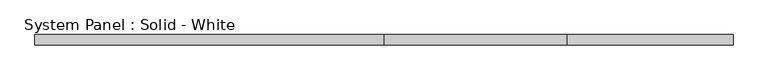
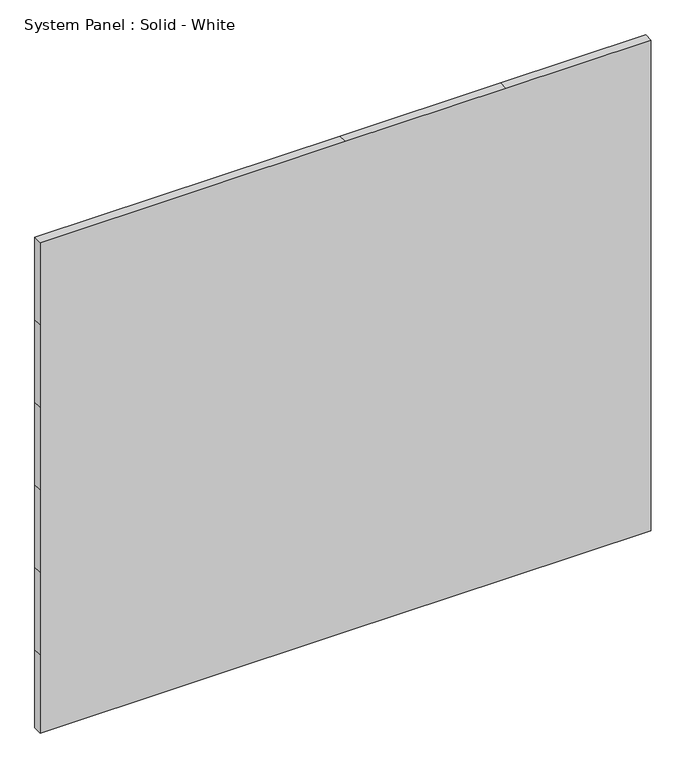
"""IFC4 building model written with IfcOpenShell, lengths in millimetres: plate geometry, System Panel : Solid - White."""

import ifcopenshell
import ifcopenshell.guid

model = None  # the IFC model being written
_history = None  # IfcOwnerHistory: only IFC2X3 demands one
_inside = {}  # id of a spatial element -> (the spatial element, [elements in it])
_under = {}  # id of a project, library or spatial element -> (it, [spatial elements below it])
_declared = {}  # id of a project -> (the project, [libraries it declares])
_typed = {}  # id of a type object -> (the type object, [elements of that type])
_made_of = {}  # id of a material, layer set ... -> (it, [elements and type objects made of it])


def new_model(schema):
    """Start an empty IFC model of exactly this schema.

    Asked for "IFC4X3", IfcOpenShell would pick the latest addendum, in which some entities
    have other attributes; the version numbers below select the first issue.
    IFC2X3 requires an IfcOwnerHistory on every rooted entity: one is made here for all.
    """
    global model, _history
    if schema == "IFC4X3":
        model = ifcopenshell.file(schema_version=(4, 3, 0, 0))
    else:
        model = ifcopenshell.file(schema=schema)
    _inside.clear()
    _under.clear()
    _declared.clear()
    _typed.clear()
    _made_of.clear()
    _history = None
    if model.schema == "IFC2X3":
        org = make("IfcOrganization", Name="unknown")
        user = make(
            "IfcPersonAndOrganization",
            ThePerson=make("IfcPerson", FamilyName="unknown"),
            TheOrganization=org,
        )
        app = make(
            "IfcApplication",
            ApplicationDeveloper=org,
            Version="unknown",
            ApplicationFullName="unknown",
            ApplicationIdentifier="unknown",
        )
        _history = make(
            "IfcOwnerHistory",
            OwningUser=user,
            OwningApplication=app,
            ChangeAction="ADDED",
            CreationDate=0,
        )
    return model


def make(cls, **values):
    """One entity of the class cls with the attributes given. An attribute that is None is left unset."""
    return model.create_entity(
        cls, **{name: value for name, value in values.items() if value is not None}
    )


def rooted(cls, **values):
    """An entity with a GlobalId (a new one), such as an element, a storey or a relation."""
    return make(cls, GlobalId=ifcopenshell.guid.new(), OwnerHistory=_history, **values)


def si_unit(unit_type, name, prefix=None):
    """IfcSIUnit, for example si_unit("LENGTHUNIT", "METRE", prefix="MILLI")."""
    return make("IfcSIUnit", UnitType=unit_type, Prefix=prefix, Name=name)


def assignment(units):
    """IfcUnitAssignment: the units of a project."""
    return None if units is None else make("IfcUnitAssignment", Units=units)


def point(xyz):
    """IfcCartesianPoint."""
    return None if xyz is None else make("IfcCartesianPoint", Coordinates=xyz)


def direction(xyz):
    """IfcDirection."""
    return None if xyz is None else make("IfcDirection", DirectionRatios=xyz)


def frame(location, z_axis=None, x_axis=None):
    """IfcAxis2Placement3D, a coordinate frame: its origin and axes. An axis left out is left unset."""
    return make(
        "IfcAxis2Placement3D",
        Location=point(location),
        Axis=direction(z_axis),
        RefDirection=direction(x_axis),
    )


def origin():
    """The frame at (0, 0, 0) with its axes left unset."""
    return frame((0.0, 0.0, 0.0))


def place(relative_to, where):
    """IfcLocalPlacement: puts the frame where relative to a parent placement (None: the world)."""
    return make(
        "IfcLocalPlacement", PlacementRelTo=relative_to, RelativePlacement=where
    )


def context(
    kind, dimensions, precision=None, world=None, true_north=None, identifier=None
):
    """IfcGeometricRepresentationContext, for example the 3D "Model" context."""
    return make(
        "IfcGeometricRepresentationContext",
        ContextIdentifier=identifier,
        ContextType=kind,
        CoordinateSpaceDimension=dimensions,
        Precision=precision,
        WorldCoordinateSystem=world,
        TrueNorth=true_north,
    )


def project(units=None, contexts=None):
    """IfcProject with its units and contexts."""
    return rooted(
        "IfcProject",
        Name="project",
        RepresentationContexts=contexts,
        UnitsInContext=assignment(units),
    )


def spatial(cls, under=None, at=None, **own):
    """A site, building, storey or space (cls), placed at a placement, below another one or the project."""
    s = rooted(cls, ObjectPlacement=at, **own)
    if under is not None:
        _under.setdefault(under.id(), (under, []))[1].append(s)
    return s


def polyline(points):
    """IfcPolyline through the points."""
    return make("IfcPolyline", Points=[point(p) for p in points])


def outline(outer, holes=None, kind="AREA"):
    """IfcArbitraryClosedProfileDef: a profile drawn as a closed curve; with holes, ...WithVoids."""
    if holes is None:
        return make("IfcArbitraryClosedProfileDef", ProfileType=kind, OuterCurve=outer)
    return make(
        "IfcArbitraryProfileDefWithVoids",
        ProfileType=kind,
        OuterCurve=outer,
        InnerCurves=holes,
    )


def extrude(swept, where, along, depth):
    """IfcExtrudedAreaSolid: the profile swept, set in the frame where, extruded along a direction by depth."""
    return make(
        "IfcExtrudedAreaSolid",
        SweptArea=swept,
        Position=where,
        ExtrudedDirection=direction(along),
        Depth=depth,
    )


def shape(context_of_items, identifier, shape_type, items):
    """IfcShapeRepresentation: the items that make up one representation, for example the "Body"."""
    return make(
        "IfcShapeRepresentation",
        ContextOfItems=context_of_items,
        RepresentationIdentifier=identifier,
        RepresentationType=shape_type,
        Items=items,
    )


def source(mapping_origin, context_of_items, identifier, shape_type, items):
    """IfcRepresentationMap: a shape defined once, which mapped items show again and again."""
    return make(
        "IfcRepresentationMap",
        MappingOrigin=mapping_origin,
        MappedRepresentation=shape(context_of_items, identifier, shape_type, items),
    )


def transform(
    local_origin,
    x_axis=None,
    y_axis=None,
    z_axis=None,
    scale=None,
    scale2=None,
    scale3=None,
    uniform=True,
):
    """IfcCartesianTransformationOperator3D, or its non-uniform kind. x_axis, y_axis, z_axis: its Axis1, 2, 3."""
    if uniform:
        return make(
            "IfcCartesianTransformationOperator3D",
            Axis1=direction(x_axis),
            Axis2=direction(y_axis),
            LocalOrigin=point(local_origin),
            Scale=scale,
            Axis3=direction(z_axis),
        )
    return make(
        "IfcCartesianTransformationOperator3DnonUniform",
        Axis1=direction(x_axis),
        Axis2=direction(y_axis),
        LocalOrigin=point(local_origin),
        Scale=scale,
        Axis3=direction(z_axis),
        Scale2=scale2,
        Scale3=scale3,
    )


def mapped(mapping_source, mapping_target):
    """IfcMappedItem: shows the shape of a source again, moved by a transform."""
    return make(
        "IfcMappedItem", MappingSource=mapping_source, MappingTarget=mapping_target
    )


def made_of(thing, what):
    """Note that an element or type object is made of a material, layer set ...; save() writes the relation."""
    if what is not None:
        _made_of.setdefault(what.id(), (what, []))[1].append(thing)
    return thing


def element(
    cls,
    number,
    at=None,
    inside=None,
    cuts=None,
    type_object=None,
    material=None,
    context=None,
    identifier="Body",
    shape_type=None,
    held_by="IfcProductDefinitionShape",
    body=None,
    shapes=None,
    **own,
):
    """One element of the class cls, such as IfcWall. Its Tag is "e" and its number.

    at: its placement. inside: the storey or other place that contains it. cuts: it is an
    opening in that element (IfcRelVoidsElement). A single representation is given by context,
    identifier, shape_type and body (its items); several are given by shapes. held_by: the class
    of the entity that holds the representations. save() writes the other relations.
    """
    e = rooted(cls, Tag="e%d" % number, ObjectPlacement=at, **own)
    if body is not None:
        shapes = [shape(context, identifier, shape_type, body)]
    if shapes is not None:
        e.Representation = make(held_by, Representations=shapes)
    if inside is not None:
        _inside.setdefault(inside.id(), (inside, []))[1].append(e)
    if cuts is not None:
        rooted(
            "IfcRelVoidsElement", RelatingBuildingElement=cuts, RelatedOpeningElement=e
        )
    if type_object is not None:
        _typed.setdefault(type_object.id(), (type_object, []))[1].append(e)
    return made_of(e, material)


def aggregate(whole, parts):
    """IfcRelAggregates: a whole, such as a stair, and the parts it consists of."""
    return rooted("IfcRelAggregates", RelatingObject=whole, RelatedObjects=parts)


def save(model, path):
    """Write the relations noted so far, then the file.

    IfcRelAggregates (storeys below a building ...), IfcRelContainedInSpatialStructure (elements
    in a storey), IfcRelDefinesByType, IfcRelAssociatesMaterial and IfcRelDeclares: one each for
    every whole, place, type object, material and project.
    """
    for whole, parts in _under.values():
        aggregate(whole, parts)
    for where, things in _inside.values():
        rooted(
            "IfcRelContainedInSpatialStructure",
            RelatedElements=things,
            RelatingStructure=where,
        )
    for kind, things in _typed.values():
        rooted("IfcRelDefinesByType", RelatedObjects=things, RelatingType=kind)
    for what, things in _made_of.values():
        rooted("IfcRelAssociatesMaterial", RelatedObjects=things, RelatingMaterial=what)
    for by, libraries in _declared.values():
        rooted("IfcRelDeclares", RelatingContext=by, RelatedDefinitions=libraries)
    model.write(path)


def system_panel_solid_white_3e93b874(model_context):
    return source(origin(), model_context, "Body", "SweptSolid", [
        extrude(outline(polyline([(0.0, -2136.3214286), (0.0, 0.0), (0.0, 1122.5892857), (0.0, 2136.3214286), (577.85, 2136.3214286), (1187.45, 2136.3214286), (1797.05, 2136.3214286), (2406.65, 2136.3214286), (3016.25, 2136.3214286), (3625.85, 2136.3214286), (3625.85, 1122.5892857), (3625.85, 0.0), (3625.85, -2136.3214286), (3016.25, -2136.3214286), (2406.65, -2136.3214286), (1797.05, -2136.3214286), (1187.45, -2136.3214286), (577.85, -2136.3214286), (0.0, -2136.3214286)])), frame((0.0, -19.05, 0.0), z_axis=(0.0, 1.0, 0.0), x_axis=(0.0, 0.0, 1.0)), (0.0, 0.0, 1.0), 63.5),
    ])


if __name__ == "__main__":
    model = new_model("IFC4")
    model_context = context("Model", 3, world=origin())
    ifc_project = project(units=[si_unit("LENGTHUNIT", "METRE", prefix="MILLI")], contexts=[model_context])
    site = spatial("IfcSite", under=ifc_project)
    building = spatial("IfcBuilding", under=site)
    placement = place(None, origin())
    system_panel_solid_white_shape = system_panel_solid_white_3e93b874(model_context)
    element("IfcPlate", 1, ObjectType="System Panel : Solid - White", at=placement, inside=building, context=model_context, shape_type="MappedRepresentation", body=[
        mapped(system_panel_solid_white_shape, transform((0.0, 0.0, 0.0), x_axis=(1.0, 0.0, 0.0), y_axis=(0.0, 1.0, 0.0), z_axis=(0.0, 0.0, 1.0))),
    ])
    save(model, "model.ifc")

# Revit data of these elements
# Project information
#   SR Document GUID = "4c5931b3-dab8-40a9-800d-cf79e49c7e77"
# Element 1 (IfcPlate, "System Panel : Solid - White")
#   Materials on its faces: "White Panel"
# Materials
#   "White Panel": class "Unassigned", colour RGB 255 255 255, transparency 0
